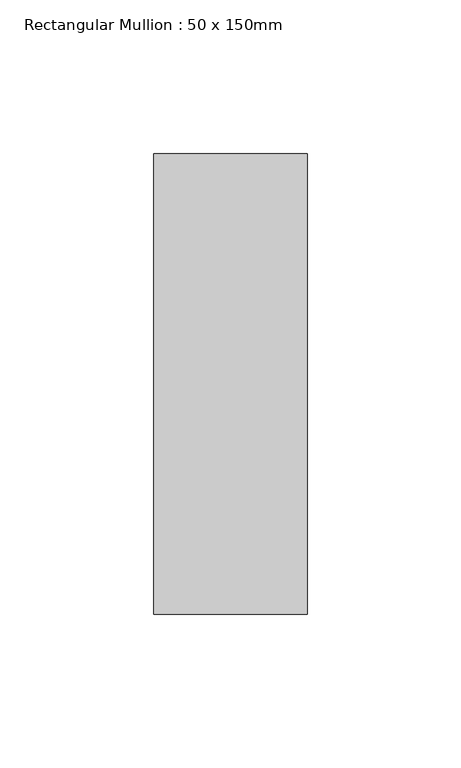
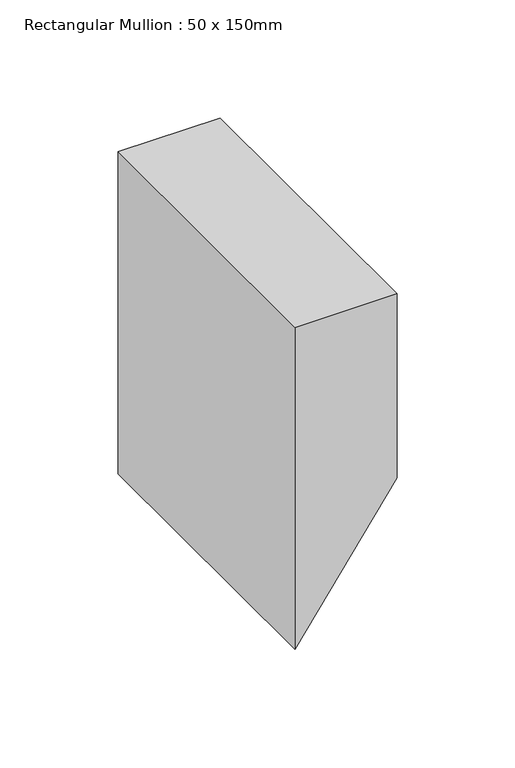
"""IFC4 building model written with IfcOpenShell, lengths in millimetres: member geometry, Rectangular Mullion : 50 x 150mm."""

from ifc_helpers import new_model, si_unit, frame, origin, place, context, project, spatial, polyline, outline, extrude, source, transform, mapped, element, save


def rectangular_mullion_50_x_150mm_544dbf8b(model_context):
    return source(origin(), model_context, "Body", "SweptSolid", [
        extrude(outline(polyline([(0.0, 25.0), (0.0, -25.0), (-166.6425563, -25.0), (-95.235156, 25.0), (0.0, 25.0)])), frame((0.0, -75.0, 0.0), z_axis=(0.0, 1.0, 0.0), x_axis=(0.0, 0.0, 1.0)), (0.0, 0.0, 1.0), 150.0),
    ])


if __name__ == "__main__":
    model = new_model("IFC4")
    model_context = context("Model", 3, world=origin())
    ifc_project = project(units=[si_unit("LENGTHUNIT", "METRE", prefix="MILLI")], contexts=[model_context])
    site = spatial("IfcSite", under=ifc_project)
    building = spatial("IfcBuilding", under=site)
    placement = place(None, origin())
    rectangular_mullion_50_x_150mm_shape = rectangular_mullion_50_x_150mm_544dbf8b(model_context)
    element("IfcMember", 1, ObjectType="Rectangular Mullion : 50 x 150mm", at=placement, inside=building, context=model_context, shape_type="MappedRepresentation", body=[
        mapped(rectangular_mullion_50_x_150mm_shape, transform((0.0, 0.0, 0.0), x_axis=(1.0, 0.0, 0.0), y_axis=(0.0, 1.0, 0.0), z_axis=(0.0, 0.0, 1.0))),
    ])
    save(model, "model.ifc")

# Revit data of these elements
# Type "Rectangular Mullion : 50 x 150mm"
#   built-in parameter 1007304 = 0.492126 (stored number, unit not read)
#   built-in parameter 1007301 = 0.082021 (stored number, unit not read)
#   built-in parameter 1007300 = 0.082021 (stored number, unit not read)
# Element 1 (IfcMember, "Rectangular Mullion : 50 x 150mm")
#   Materials on its faces: "Aluminium"
# Materials
#   "Aluminium": class "Metal", colour RGB 247 247 247, transparency 0, Description = "Aluminium 6061", Cost = 0
